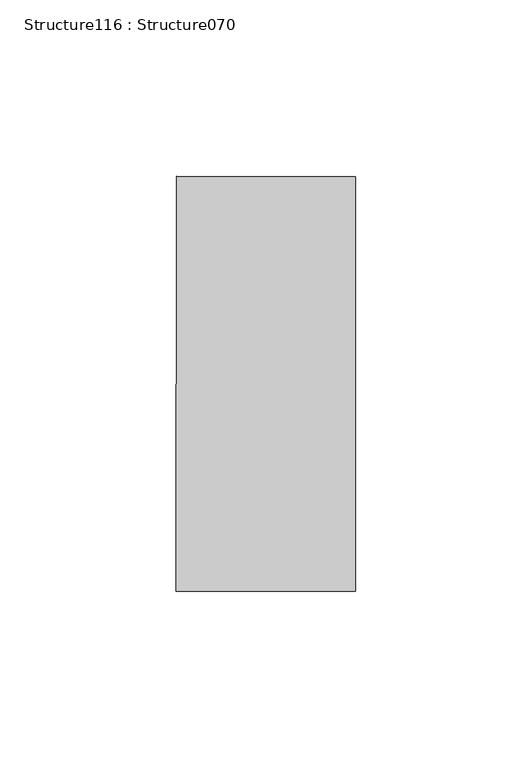
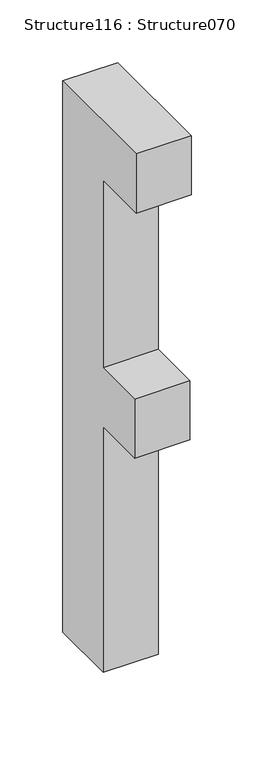
"""IFC4 building model written with IfcOpenShell, lengths in millimetres: proxy geometry, Structure116 : Structure070."""

from ifc_helpers import new_model, si_unit, frame, origin, place, context, project, spatial, polyline, outline, extrude, source, transform, mapped, element, save


def structure116_structure070_deba5427(model_context):
    return source(origin(), model_context, "Body", "SweptSolid", [
        extrude(outline(polyline([(537.7810299, 0.0), (537.7810299, -117.5476552), (480.1634256, -117.5476552), (480.1634256, -64.5410676), (297.3185942, -64.5410676), (297.3185942, -115.249797), (239.6949411, -115.249797), (239.6949411, -64.5410676), (0.0, -64.5410676), (0.0, 0.0), (537.7810299, 0.0)])), frame((-56111.4726568, 291370.7634506, -166.7961167), z_axis=(-0.9999998917542984, 0.00046528635450596156, 0.0), x_axis=(0.0, 0.0, 1.0)), (0.0, 0.0, 1.0), 50.8),
    ])


if __name__ == "__main__":
    model = new_model("IFC4")
    model_context = context("Model", 3, world=origin())
    ifc_project = project(units=[si_unit("LENGTHUNIT", "METRE", prefix="MILLI")], contexts=[model_context])
    site = spatial("IfcSite", under=ifc_project)
    building = spatial("IfcBuilding", under=site)
    placement = place(None, origin())
    structure116_structure070_shape = structure116_structure070_deba5427(model_context)
    element("IfcBuildingElementProxy", 1, Name="Structure116 : Structure070", ObjectType="Structure116 : Structure070", at=placement, inside=building, context=model_context, shape_type="MappedRepresentation", body=[
        mapped(structure116_structure070_shape, transform((0.0, 0.0, 0.0), x_axis=(1.0, 0.0, 0.0), y_axis=(0.0, 1.0, 0.0), z_axis=(0.0, 0.0, 1.0))),
    ])
    save(model, "model.ifc")

# Revit data of these elements
# Type "Structure116 : Structure070"
#   NameOverride = "Structure070"
# Element 1 (IfcBuildingElementProxy, "Structure116 : Structure070")
#   Materials on its faces: "BRUSHED ALUMINUM LETTERING"
# Materials
#   "BRUSHED ALUMINUM LETTERING": class "Unassigned", colour RGB 169 181 186, transparency 0, Cost = 0
